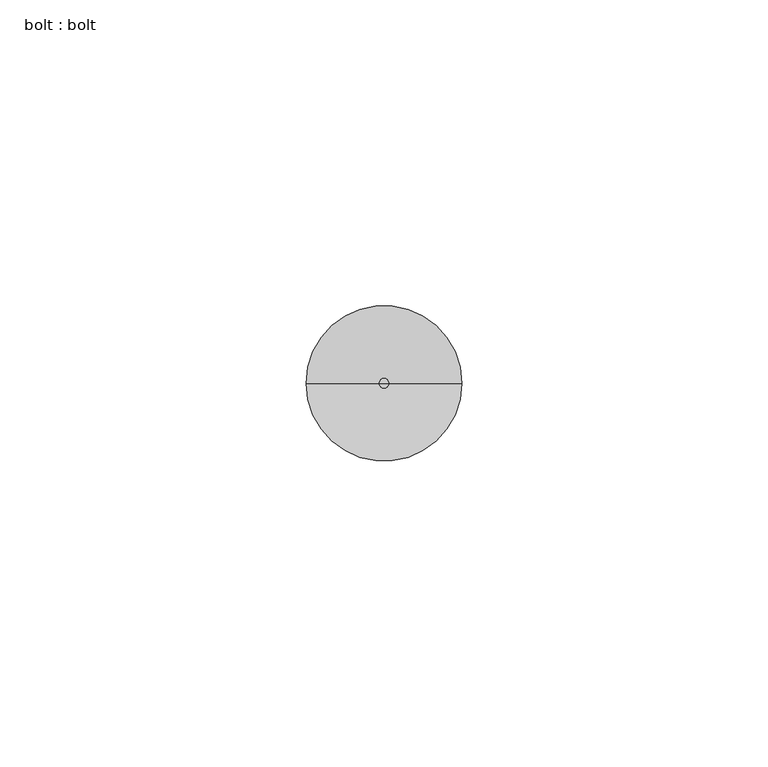
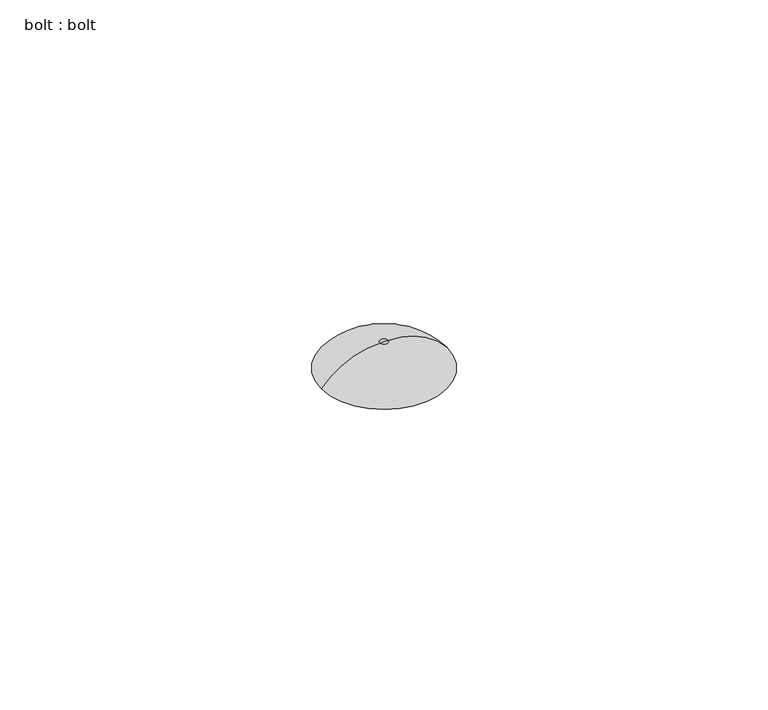
"""IFC4 building model written with IfcOpenShell, lengths in millimetres: proxy geometry, bolt : bolt."""

from ifc_helpers import new_model, si_unit, point, frame, origin, place, context, project, spatial, circle_curve, ellipse_curve, trimmed, source, transform, mapped, element, save
from ifc_brep_helpers import plane_surface, revolved_surface, advanced_brep


def bolt_bolt_898a474d(model_context):
    return source(origin(), model_context, "Body", "AdvancedBrep", [
        advanced_brep(
        [(0.0, 0.0, 0.0), (-12.7, 0.0, 0.0), (12.7, 0.0, 0.0), (0.79375, 0.0, 5.6544043), (-0.79375, 0.0, 5.6544043), (0.0, 0.0, 5.6544043)],
        [
            (0, 1),
            (1, 2, circle_curve(frame((0.0, 0.0, 0.0), z_axis=(0.0, 0.0, -1.0), x_axis=(-1.0, 0.0, 0.0)), 12.7)),
            (2, 0),
            (2, 1, circle_curve(frame((0.0, 0.0, 0.0), z_axis=(0.0, 0.0, -1.0), x_axis=(-1.0, 0.0, 0.0)), 12.7)),
            (3, 4, circle_curve(frame((0.0, 0.0, 5.6544043), z_axis=(0.0, 0.0, 1.0), x_axis=(-1.0, 0.0, 0.0)), 0.79375)),
            (4, 5),
            (5, 3),
            (4, 3, circle_curve(frame((0.0, 0.0, 5.6544043), z_axis=(0.0, 0.0, 1.0), x_axis=(-1.0, 0.0, 0.0)), 0.79375)),
            (1, 4, circle_curve(frame((-0.79375, 0.0, -9.7080519), z_axis=(0.0, 1.0, 0.0), x_axis=(1.0, 0.0, 0.0)), 15.3624562)),
            (3, 2, circle_curve(frame((0.79375, 0.0, -9.7080519), z_axis=(0.0, 1.0, 0.0), x_axis=(-1.0, 0.0, 0.0)), 15.3624562)),
        ],
        [
            plane_surface(frame((0.0, 0.0, 0.0), z_axis=(0.0, 0.0, -1.0), x_axis=(-1.0, 0.0, 0.0))),
            plane_surface(frame((0.0, 0.0, 5.6544043), z_axis=(0.0, 0.0, 1.0), x_axis=(-1.0, 0.0, 0.0))),
            revolved_surface(trimmed(ellipse_curve(frame((-0.79375, 0.0, -9.7080519), z_axis=(0.0, -1.0, 0.0), x_axis=(1.0, 0.0, 0.0)), 15.3624562, 15.3624562), [point((-0.79375, 0.0, 5.6544043))], [point((-12.7, 0.0, 0.0))], True, "CARTESIAN"), (0.0, 0.0, 12.7), (0.0, 0.0, -1.0)),
        ],
        [
            (0, [[1, 2, 3]]),
            (0, [[-3, 4, -1]]),
            (1, [[5, 6, 7]]),
            (1, [[8, -7, -6]]),
            (2, [[-2, 9, -5, 10]]),
            (2, [[-4, -10, -8, -9]]),
        ],
    ),
    ])


if __name__ == "__main__":
    model = new_model("IFC4")
    model_context = context("Model", 3, world=origin())
    ifc_project = project(units=[si_unit("LENGTHUNIT", "METRE", prefix="MILLI")], contexts=[model_context])
    site = spatial("IfcSite", under=ifc_project)
    building = spatial("IfcBuilding", under=site)
    placement = place(None, origin())
    bolt_bolt_shape = bolt_bolt_898a474d(model_context)
    element("IfcBuildingElementProxy", 1, Name="bolt : bolt", ObjectType="bolt : bolt", at=placement, inside=building, context=model_context, shape_type="MappedRepresentation", body=[
        mapped(bolt_bolt_shape, transform((0.0, 0.0, 0.0), x_axis=(1.0, 0.0, 0.0), y_axis=(0.0, 1.0, 0.0), z_axis=(0.0, 0.0, 1.0))),
    ])
    save(model, "model.ifc")

# Revit data of these elements
# Type "bolt : bolt"
#   Default Elevation = 4' - 0"
#   material = DECORATIVE FASTENERS (T.B.D)
# Element 1 (IfcBuildingElementProxy, "bolt : bolt")
#   Materials on its faces: "DECORATIVE FASTENERS (T.B.D)"
# Materials
#   "DECORATIVE FASTENERS (T.B.D)": class "Generic", colour RGB 61 60 59, transparency 0, Cost = 0
